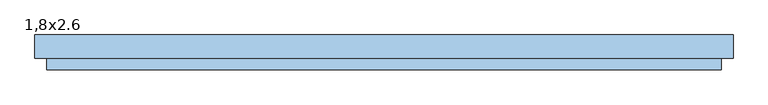
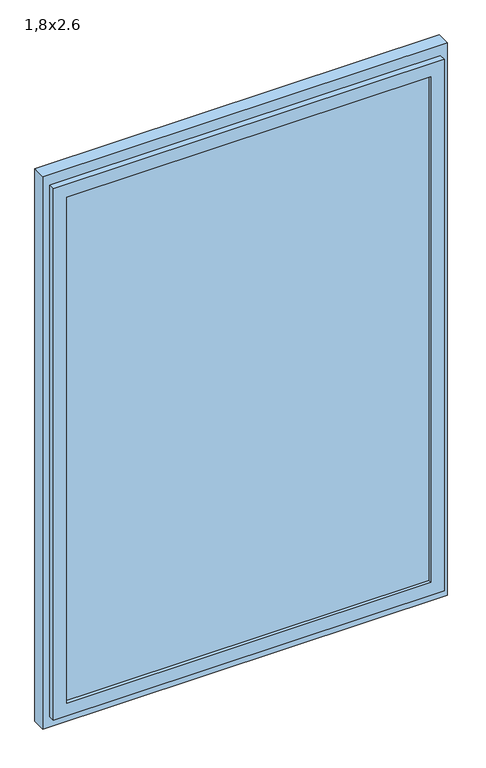
"""IFC4 building model written with IfcOpenShell, lengths in millimetres: window geometry, Fenstertür 1-flg : 1,8x2.6."""

from ifc_helpers import new_model, si_unit, frame, origin, place, context, project, spatial, polyline, outline, extrude, faceted_brep, source, transform, mapped, element, save


def window_1_8x2_6_16ffd7c0(model_context):
    return source(origin(), model_context, "Body", "SolidModel", [
        extrude(outline(polyline([(2600.0, 900.0), (2600.0, -900.0), (0.0, -900.0), (0.0, 900.0), (2600.0, 900.0)]), holes=[polyline([(2520.0, 840.0), (80.0, 840.0), (80.0, -840.0), (2520.0, -840.0), (2520.0, 840.0)])]), frame((0.0, 20.0, 0.0), z_axis=(0.0, 1.0, 0.0), x_axis=(0.0, 0.0, 1.0)), (0.0, 0.0, 1.0), 60.0),
        faceted_brep([(870.0, 20.0, 2550.0), (870.0, -10.0, 2550.0), (870.0, -10.0, 50.0), (870.0, 20.0, 50.0), (-870.0, -10.0, 2550.0), (-870.0, -10.0, 50.0), (810.0, -10.0, 110.0), (-810.0, -10.0, 110.0), (-810.0, -10.0, 2490.0), (810.0, -10.0, 2490.0), (-870.0, 20.0, 50.0), (-870.0, 20.0, 2550.0), (840.0, 20.0, 2520.0), (-840.0, 20.0, 2520.0), (-840.0, 20.0, 80.0), (840.0, 20.0, 80.0), (840.0, 50.0, 2520.0), (840.0, 50.0, 80.0), (-840.0, 50.0, 80.0), (-840.0, 50.0, 2520.0), (810.0, 50.0, 2490.0), (-810.0, 50.0, 2490.0), (-810.0, 50.0, 110.0), (810.0, 50.0, 110.0)], [[[0, 1, 2, 3]], [[1, 4, 5, 2], [6, 7, 8, 9]], [[3, 2, 5, 10]], [[3, 10, 11, 0], [12, 13, 14, 15]], [[16, 12, 15, 17]], [[17, 15, 14, 18]], [[17, 18, 19, 16], [20, 21, 22, 23]], [[9, 20, 23, 6]], [[6, 23, 22, 7]], [[10, 5, 4, 11]], [[18, 14, 13, 19]], [[7, 22, 21, 8]], [[11, 4, 1, 0]], [[19, 13, 12, 16]], [[8, 21, 20, 9]]]),
        extrude(outline(polyline([(810.0, 5.0), (-810.0, 5.0), (-810.0, 35.0), (810.0, 35.0), (810.0, 5.0)])), frame((0.0, 0.0, 110.0), z_axis=(0.0, 0.0, 1.0), x_axis=(1.0, 0.0, 0.0)), (0.0, 0.0, 1.0), 2380.0),
    ])


if __name__ == "__main__":
    model = new_model("IFC4")
    model_context = context("Model", 3, world=origin())
    ifc_project = project(units=[si_unit("LENGTHUNIT", "METRE", prefix="MILLI")], contexts=[model_context])
    site = spatial("IfcSite", under=ifc_project)
    building = spatial("IfcBuilding", under=site)
    placement = place(None, origin())
    window_1_8x2_6_shape = window_1_8x2_6_16ffd7c0(model_context)
    element("IfcWindow", 1, ObjectType="Fenstertür 1-flg : 1,8x2.6", at=placement, inside=building, context=model_context, shape_type="MappedRepresentation", body=[
        mapped(window_1_8x2_6_shape, transform((0.0, 0.0, 0.0), x_axis=(1.0, 0.0, 0.0), y_axis=(0.0, 1.0, 0.0), z_axis=(0.0, 0.0, 1.0))),
    ])
    save(model, "model.ifc")

# Revit data of these elements
# Type "Fenstertür 1-flg : 1,8x2.6"
#   Type Mark = "70"
#   Operation = "SinglePanel"
#   Construction Type Id = "GSP4R"
#   Keynote = "16.05.01"
#   Analytic Construction = "1/8 Zoll Pilkington-Verglasung einfach"
#   Visual Light Transmittance = 0.9
#   Thermal Resistance (R) = 0.1491 (m²·K)/W
#   Solar Heat Gain Coefficient = 0.86
#   Rough Width = 1.800 m
#   Rough Height = 2.600 m
#   Heat Transfer Coefficient (U) = 6.7069 W/(m²·K)
#   Rahmentiefe = 0.060 m
#   Rahmenhöhe - unten = 0.080 m
#   Rahmenhöhe - oben = 0.080 m
#   Rahmenbreite = 0.060 m
#   Height = 2.600 m
#   Tiefe Flügel = 0.060 m
#   Flügelbreite = 0.060 m
#   Einbautiefe (von außen) [instance default] = 0.080 m
#   Width = 1.800 m
#   Kippflügel [instance default] = yes
#   Drehflügel im Grundriss darstellen [instance default] = yes
#   Drehflügel 1 [instance default] = yes
#   Rahmen 1 [instance default] = none
#   Glas [instance default] = none
#   Flügel [instance default] = none
#   Fensterbank Außenseite [instance default] = none
#   Wall Closure = (empty or 0)
# Element 1 (IfcWindow, "Fenstertür 1-flg : 1,8x2.6")
#   Einbautiefe (von außen) = 0.230 m
#   Materials on its faces: "Kunststoff - Weiß", "Glas"
# Materials
#   "Kunststoff - Weiß": class "Kunststoff", colour RGB 249 249 249, transparency 0, Cost = 0
#   "Glas": class "Glas", colour RGB 0 0 255, transparency 0.75, Comments = "Render-Darstellung nicht aktualisiert ", Cost = 0
